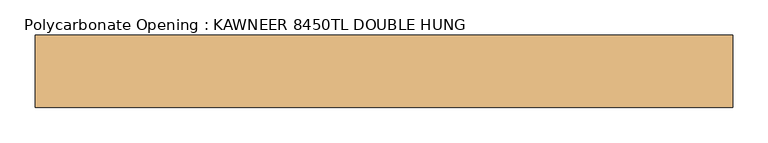
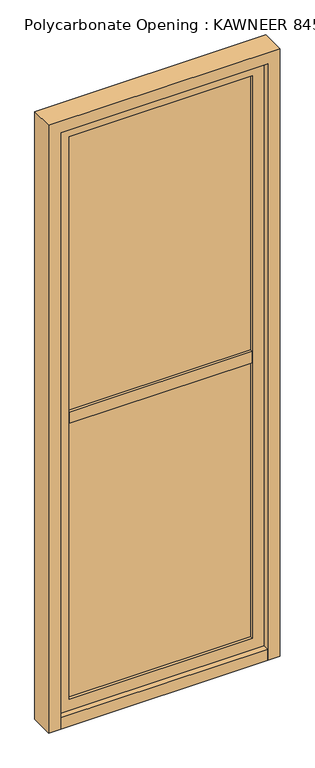
"""IFC4 building model written with IfcOpenShell, lengths in millimetres: door geometry, Polycarbonate Opening : KAWNEER 8450TL DOUBLE HUNG."""

from ifc_helpers import new_model, si_unit, frame, origin, origin_with_axes, place, context, project, spatial, polyline, outline, extrude, source, transform, mapped, element, save


def polycarbonate_opening_kawneer_8450tl_double_hung_046086d1(model_context):
    return source(origin(), model_context, "Body", "SweptSolid", [
        extrude(outline(polyline([(440.1908884, 12.7), (440.1908884, -12.7), (-440.1908884, -12.7), (-440.1908884, 12.7), (440.1908884, 12.7)])), frame((0.0, 0.0, 50.8), z_axis=(0.0, 0.0, 1.0), x_axis=(1.0, 0.0, 0.0)), (0.0, 0.0, 1.0), 2625.4648118),
        extrude(outline(polyline([(2676.2648118, -440.1908884), (0.0, -440.1908884), (0.0, 440.1908884), (2676.2648118, 440.1908884), (2676.2648118, -440.1908884)]), holes=[polyline([(101.6, 389.3908884), (101.6, -389.3908884), (2625.4648118, -389.3908884), (2625.4648118, 389.3908884), (101.6, 389.3908884)])]), frame((0.0, -25.4, 0.0), z_axis=(0.0, 1.0, 0.0), x_axis=(0.0, 0.0, 1.0)), (0.0, 0.0, 1.0), 50.8),
        extrude(outline(polyline([(2727.0648118, 490.9908884), (2727.0648118, -490.9908884), (0.0, -490.9908884), (0.0, -440.1908884), (2676.2648118, -440.1908884), (2676.2648118, 440.1908884), (0.0, 440.1908884), (0.0, 490.9908884), (2727.0648118, 490.9908884)])), frame((0.0, -50.8, 0.0), z_axis=(0.0, 1.0, 0.0), x_axis=(0.0, 0.0, 1.0)), (0.0, 0.0, 1.0), 101.6),
        extrude(outline(polyline([(389.3908884, 25.4), (389.3908884, -25.4), (-389.3908884, -25.4), (-389.3908884, 25.4), (389.3908884, 25.4)])), frame((0.0, 0.0, 1338.1324059), z_axis=(0.0, 0.0, 1.0), x_axis=(1.0, 0.0, 0.0)), (0.0, 0.0, 1.0), 50.8),
        extrude(outline(polyline([(440.1908884, 50.8), (440.1908884, -50.8), (-440.1908884, -50.8), (-440.1908884, 50.8), (440.1908884, 50.8)])), origin_with_axes(), (0.0, 0.0, 1.0), 50.8),
    ])


if __name__ == "__main__":
    model = new_model("IFC4")
    model_context = context("Model", 3, world=origin())
    ifc_project = project(units=[si_unit("LENGTHUNIT", "METRE", prefix="MILLI")], contexts=[model_context])
    site = spatial("IfcSite", under=ifc_project)
    building = spatial("IfcBuilding", under=site)
    placement = place(None, origin())
    polycarbonate_opening_kawneer_8450tl_double_hung_shape = polycarbonate_opening_kawneer_8450tl_double_hung_046086d1(model_context)
    element("IfcDoor", 1, ObjectType="Polycarbonate Opening : KAWNEER 8450TL DOUBLE HUNG", at=placement, inside=building, context=model_context, shape_type="MappedRepresentation", body=[
        mapped(polycarbonate_opening_kawneer_8450tl_double_hung_shape, transform((0.0, 0.0, 0.0), x_axis=(1.0, 0.0, 0.0), y_axis=(0.0, 1.0, 0.0), z_axis=(0.0, 0.0, 1.0))),
    ])
    save(model, "model.ifc")

# Revit data of these elements
# Type "Polycarbonate Opening : KAWNEER 8450TL DOUBLE HUNG"
#   Type Mark = "59"
#   OD_DS_Door_Material = "ALUM./GLAZING"
#   OD_DS_Door_Type = "STOREFRONT - DOUBLE HUNG WINDOW"
#   OD_DS_Lockset = "POLE OPERATOR HARDWARE FOR TOP SASH; BOTTOM SASH MECHANICALLY FIXED"
#   Analytic Construction = "<None>"
#   offset [instance default] = 0' - 2"
#   Stile = 0' - 2"
#   Mullion Width = 0' - 2"
#   Mullion Depth = 0' - 4"
#   Opening Size [instance default] = 5' - 1.50212"
#   Door Width [instance default] = 5' - 1.50212"
#   Window ON/OFF = no
#   Door On/Off = yes
#   Mullion Material = DOUBLE HUNG (CLEAR ANODIZED ALUM) - TEMPERED INSULATED GLAZING (CARDINAL GLASS LoĒ²-240\nOR EQUIVALENT)
#   Glass Material = TEMPERED INSULATED GLAZING (CARDINAL GLASS LoĒ²-240\nOR EQUIVALENT)
#   Door Material = DOUBLE HUNG (CLEAR ANODIZED ALUM) - TEMPERED INSULATED GLAZING (CARDINAL GLASS LoĒ²-240\nOR EQUIVALENT)
# Element 1 (IfcDoor, "Polycarbonate Opening : KAWNEER 8450TL DOUBLE HUNG")
#   offset = 0' - 0"
#   Materials on its faces: "DOUBLE HUNG (CLEAR ANODIZED ALUM) - TEMPERED INSULATED GLAZING (CARDINAL GLASS LoĒ²-240\nOR EQUIVALENT)", "TEMPERED INSULATED GLAZING (CARDINAL GLASS LoĒ²-240\nOR EQUIVALENT)"
# Materials
#   "DOUBLE HUNG (CLEAR ANODIZED ALUM) - TEMPERED INSULATED GLAZING (CARDINAL GLASS LoĒ²-240\nOR EQUIVALENT)": class "Metal", colour RGB 244 244 244, transparency 0, Description = "Aluminum 6061", Cost = 0
#   "TEMPERED INSULATED GLAZING (CARDINAL GLASS LoĒ²-240\nOR EQUIVALENT)": class "Glass", colour RGB 196 205 210, transparency 0.85, Description = "Soda Lime Glass", Cost = 0
